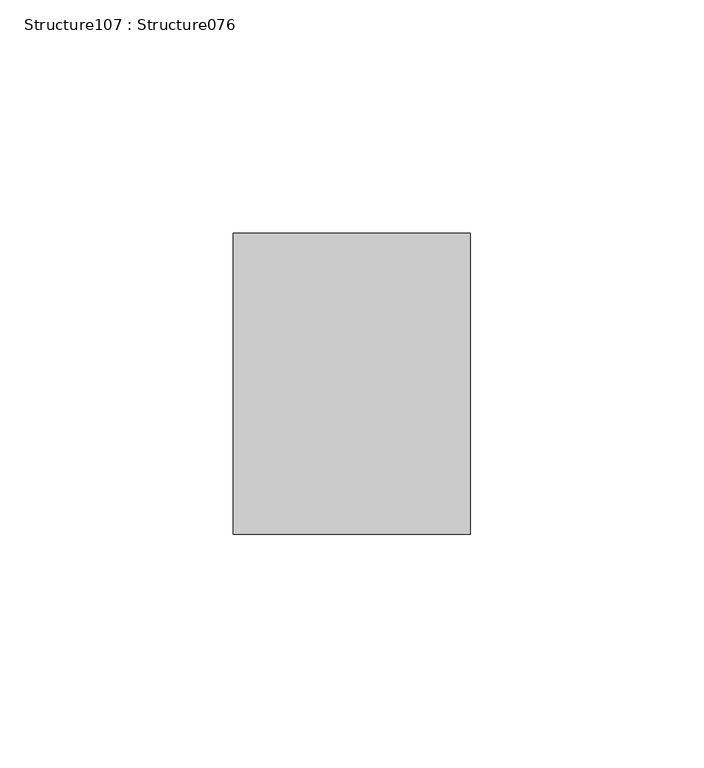
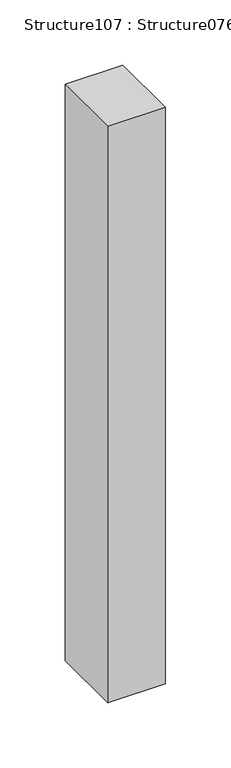
"""IFC4 building model written with IfcOpenShell, lengths in millimetres: proxy geometry, Structure107 : Structure076."""

from ifc_helpers import new_model, si_unit, frame, origin, place, context, project, spatial, polyline, outline, extrude, source, transform, mapped, element, save


def structure107_structure076_69120e6c(model_context):
    return source(origin(), model_context, "Body", "SweptSolid", [
        extrude(outline(polyline([(-56162.4016978, 291093.4386833), (-56162.3716677, 291157.979744), (-56111.5716732, 291157.9561074), (-56111.6017033, 291093.4150468), (-56162.4016978, 291093.4386833)])), frame((0.0, 0.0, -166.7961167), z_axis=(0.0, 0.0, 1.0), x_axis=(1.0, 0.0, 0.0)), (0.0, 0.0, 1.0), 537.7810299),
    ])


if __name__ == "__main__":
    model = new_model("IFC4")
    model_context = context("Model", 3, world=origin())
    ifc_project = project(units=[si_unit("LENGTHUNIT", "METRE", prefix="MILLI")], contexts=[model_context])
    site = spatial("IfcSite", under=ifc_project)
    building = spatial("IfcBuilding", under=site)
    placement = place(None, origin())
    structure107_structure076_shape = structure107_structure076_69120e6c(model_context)
    element("IfcBuildingElementProxy", 1, Name="Structure107 : Structure076", ObjectType="Structure107 : Structure076", at=placement, inside=building, context=model_context, shape_type="MappedRepresentation", body=[
        mapped(structure107_structure076_shape, transform((0.0, 0.0, 0.0), x_axis=(1.0, 0.0, 0.0), y_axis=(0.0, 1.0, 0.0), z_axis=(0.0, 0.0, 1.0))),
    ])
    save(model, "model.ifc")

# Revit data of these elements
# Type "Structure107 : Structure076"
#   NameOverride = "Structure076"
# Element 1 (IfcBuildingElementProxy, "Structure107 : Structure076")
#   Materials on its faces: "BRUSHED ALUMINUM LETTERING"
# Materials
#   "BRUSHED ALUMINUM LETTERING": class "Unassigned", colour RGB 169 181 186, transparency 0, Cost = 0
